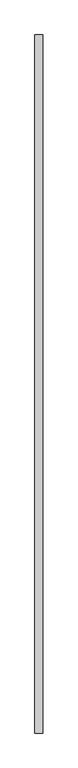
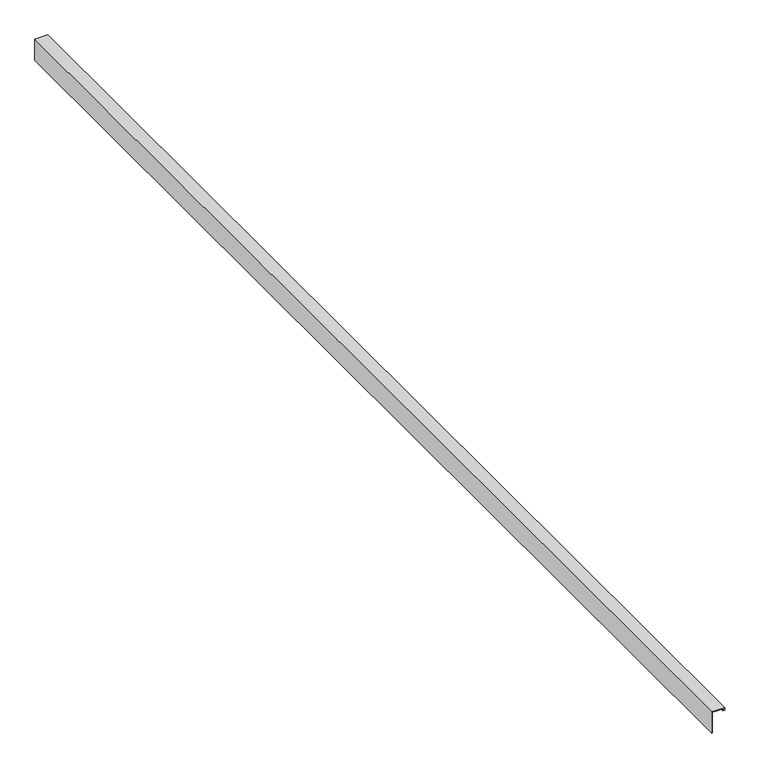
"""IFC4 building model written with IfcOpenShell, lengths in millimetres: proxy geometry, GRAVEL STOP14:GRAVEL STOP003:305306 : GRAVEL STOP14:GRAVEL STOP003:305306."""

from ifc_helpers import new_model, si_unit, frame, origin, place, context, project, spatial, polyline, outline, extrude, source, transform, mapped, element, save


def generic_models_96f309f1(model_context):
    return source(origin(), model_context, "Body", "SweptSolid", [
        extrude(outline(polyline([(40197.5761757, 398.6551832), (40234.4061757, 398.6551832), (40234.4061757, 418.3401832), (40232.1963757, 418.3401832), (40232.1963757, 416.6077268), (40230.9263757, 416.6077268), (40230.9263757, 419.6101832), (40235.6761757, 419.6101832), (40235.6761757, 397.3851832), (40197.5761757, 397.3851832), (40197.5761757, 398.6551832)])), frame((0.0, -774.5581162, 0.0), z_axis=(0.0, 1.0, 0.0), x_axis=(0.0, 0.0, 1.0)), (0.0, 0.0, 1.0), 2000.25),
    ])


if __name__ == "__main__":
    model = new_model("IFC4")
    model_context = context("Model", 3, world=origin())
    ifc_project = project(units=[si_unit("LENGTHUNIT", "METRE", prefix="MILLI")], contexts=[model_context])
    site = spatial("IfcSite", under=ifc_project)
    building = spatial("IfcBuilding", under=site)
    placement = place(None, origin())
    generic_models_shape = generic_models_96f309f1(model_context)
    element("IfcBuildingElementProxy", 1, Name="GRAVEL STOP14:GRAVEL STOP003:305306 : GRAVEL STOP14:GRAVEL STOP003:305306", ObjectType="GRAVEL STOP14:GRAVEL STOP003:305306 : GRAVEL STOP14:GRAVEL STOP003:305306", at=placement, inside=building, context=model_context, shape_type="MappedRepresentation", body=[
        mapped(generic_models_shape, transform((0.0, 0.0, 0.0), x_axis=(1.0, 0.0, 0.0), y_axis=(0.0, 1.0, 0.0), z_axis=(0.0, 0.0, 1.0))),
    ])
    save(model, "model.ifc")

# Revit data of these elements
# Type "GRAVEL STOP14:GRAVEL STOP003:305306 : GRAVEL STOP14:GRAVEL STOP003:305306"
#   NameOverride = "GRAVEL STOP14:GRAVEL STOP003:305306"
#   ObjectTypeOverride = "GRAVEL STOP14:GRAVEL STOP003"
#   Reference = "GRAVEL STOP003"
#   Category = "Generic Models"
#   Tag = "305306"
# Element 1 (IfcBuildingElementProxy, "GRAVEL STOP14:GRAVEL STOP003:305306 : GRAVEL STOP14:GRAVEL STOP003:305306")
#   Materials on its faces: "COPPER STUCCO J BEAD"
# Materials
#   "COPPER STUCCO J BEAD": class "Unassigned", colour RGB 251 232 155, transparency 0, Cost = 0
